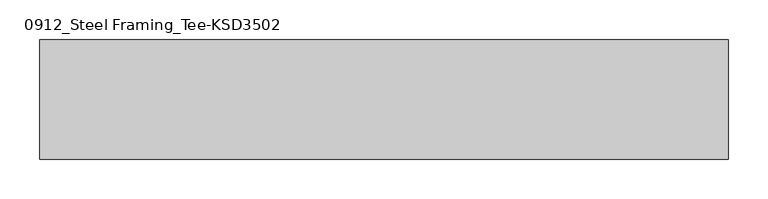
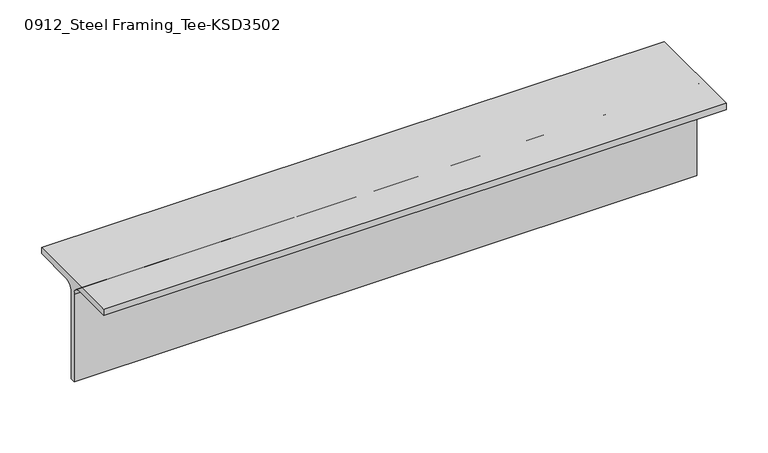
"""IFC4 building model written with IfcOpenShell, lengths in millimetres: member geometry, 0912_Steel Framing_Tee-KSD3502 : H_SB_ASB_CT-150x150x6.5x9."""

from ifc_helpers import new_model, si_unit, point, frame, frame_2d, origin, place, context, project, spatial, polyline, circle_curve, trimmed, segment, composite_curve, outline, extrude, source, transform, mapped, element, save


def member_0912_steel_framing_tee_ksd3502_70422fc5(model_context):
    return source(origin(), model_context, "Body", "SweptSolid", [
        extrude(outline(composite_curve([segment(polyline([(75.0, 75.0), (75.0, 66.0), (16.25, 66.0)]), True, "CONTINUOUS"), segment(trimmed(circle_curve(frame_2d((16.25, 53.0)), 13.0), [point((16.25, 66.0))], [point((3.25, 53.0))], True, "CARTESIAN"), True, "CONTINUOUS"), segment(polyline([(3.25, 53.0), (3.25, -75.0), (-3.25, -75.0), (-3.25, 53.0)]), True, "CONTINUOUS"), segment(trimmed(circle_curve(frame_2d((-16.25, 53.0)), 13.0), [point((-3.25, 53.0))], [point((-16.25, 66.0))], True, "CARTESIAN"), True, "CONTINUOUS"), segment(polyline([(-16.25, 66.0), (-75.0, 66.0), (-75.0, 75.0), (75.0, 75.0)]), True, "CONTINUOUS")], self_intersect=False)), frame((-365.9, 0.0, 0.0), z_axis=(1.0, 0.0, 0.0), x_axis=(0.0, 1.0, 0.0)), (0.0, 0.0, 1.0), 865.9),
    ])


if __name__ == "__main__":
    model = new_model("IFC4")
    model_context = context("Model", 3, world=origin())
    ifc_project = project(units=[si_unit("LENGTHUNIT", "METRE", prefix="MILLI")], contexts=[model_context])
    site = spatial("IfcSite", under=ifc_project)
    building = spatial("IfcBuilding", under=site)
    placement = place(None, origin())
    member_0912_steel_framing_tee_ksd3502_shape = member_0912_steel_framing_tee_ksd3502_70422fc5(model_context)
    element("IfcMember", 1, ObjectType="0912_Steel Framing_Tee-KSD3502 : H_SB_ASB_CT-150x150x6.5x9", at=placement, inside=building, context=model_context, shape_type="MappedRepresentation", body=[
        mapped(member_0912_steel_framing_tee_ksd3502_shape, transform((0.0, 0.0, 0.0), x_axis=(1.0, 0.0, 0.0), y_axis=(0.0, 1.0, 0.0), z_axis=(0.0, 0.0, 1.0))),
    ])
    save(model, "model.ifc")

# Revit data of these elements
# Type "0912_Steel Framing_Tee-KSD3502 : H_SB_ASB_CT-150x150x6.5x9"
#   H_WM Code_1 = "S01AA003-00001 | Main Steel Structure Fabrication Work | Shelter/Building | Light Steel - Standard (30KG/M>Weight) | Material: (   )"
#   H_WM Code_2 = "S03AA029-00001 | Main Steel Structure Erection Work | Shelter/Building | Light Steel (30KG/M>Weight) | Material: (   )"
#   H_WM Code_3 = "S01AA010-00001 | Main Steel Structure Fabrication Work | Shelter/Building | Steel Painting/Coating | for Non-Fireproofed Steel Surface, Surface Preparation, Primer, Second & Final Coat | Material: (   )"
#   H_Q'ty Cal Type Tag = "SB-Q2"
#   Width = 15.0 cm
#   Web Thickness = 0.65 cm
#   Web Fillet = 1.3 cm
#   Section Area = 23.39 cm²
#   Perimeter = 0.60 m²/m
#   Nominal Weight = 18.40 kgf/m
#   Height = 15.0 cm
#   Flange Thickness = 0.9 cm
#   Centroid Vertical = 7.5 cm
#   Centroid Horizontal = 7.5 cm
#   Length [instance default] = 1.5000 m
#   Structural Material [instance default] = Steel, 45-345
#   Warping Constant = (empty or 0)
#   Torsional Moment of Inertia = 0
#   Section Name Key = ""
#   Plastic Modulus weak axis = 0
#   Plastic Modulus strong axis = 0
#   Moment of Inertia weak axis = 0
#   Moment of Inertia strong axis = 0
#   Elastic Modulus weak axis = 0
#   Elastic Modulus strong axis = 0
#   Bolt Spacing = 0
#   Assembly Code = ""
# Element 1 (IfcMember, "0912_Steel Framing_Tee-KSD3502 : H_SB_ASB_CT-150x150x6.5x9")
#   Structural Material = none
# Materials
#   "Steel, 45-345": class "Metal", colour RGB 189 187 185, transparency 0, Description = "Steel 345 MPa", Cost = 0
